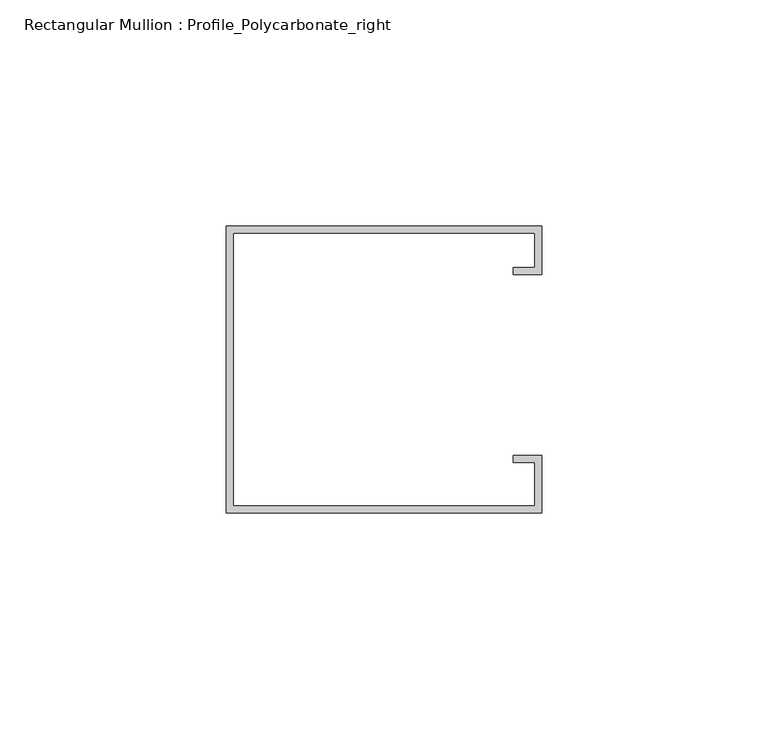
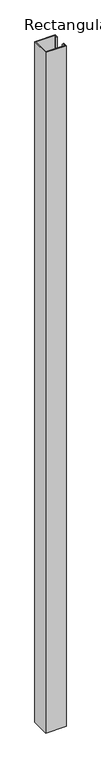
"""IFC4 building model written with IfcOpenShell, lengths in millimetres: member geometry, Rectangular Mullion : Profile_Polycarbonate_right."""

from ifc_helpers import new_model, si_unit, frame, origin, place, context, project, spatial, polyline, outline, extrude, source, transform, mapped, element, save


def rectangular_mullion_profile_polycarbonate_right_a2a6d842(model_context):
    return source(origin(), model_context, "Body", "SweptSolid", [
        extrude(outline(polyline([(0.0, -32.7), (0.0, 30.8), (69.85, 30.8), (69.85, 20.0), (63.5, 20.0), (63.5, 21.5875), (68.2625, 21.5875), (68.2625, 29.2125), (1.5875, 29.2125), (1.5875, -31.1125), (68.2625, -31.1125), (68.2625, -21.5875), (63.5, -21.5875), (63.5, -20.0), (69.85, -20.0), (69.85, -32.7), (0.0, -32.7)])), frame((0.0, 0.0, -2461.6132885), z_axis=(0.0, 0.0, 1.0), x_axis=(1.0, 0.0, 0.0)), (0.0, 0.0, 1.0), 2461.6132885),
    ])


if __name__ == "__main__":
    model = new_model("IFC4")
    model_context = context("Model", 3, world=origin())
    ifc_project = project(units=[si_unit("LENGTHUNIT", "METRE", prefix="MILLI")], contexts=[model_context])
    site = spatial("IfcSite", under=ifc_project)
    building = spatial("IfcBuilding", under=site)
    placement = place(None, origin())
    rectangular_mullion_profile_polycarbonate_right_shape = rectangular_mullion_profile_polycarbonate_right_a2a6d842(model_context)
    element("IfcMember", 1, ObjectType="Rectangular Mullion : Profile_Polycarbonate_right", at=placement, inside=building, context=model_context, shape_type="MappedRepresentation", body=[
        mapped(rectangular_mullion_profile_polycarbonate_right_shape, transform((0.0, 0.0, 0.0), x_axis=(1.0, 0.0, 0.0), y_axis=(0.0, 1.0, 0.0), z_axis=(0.0, 0.0, 1.0))),
    ])
    save(model, "model.ifc")

# Revit data of these elements
# Type "Rectangular Mullion : Profile_Polycarbonate_right"
#   built-in parameter 1007322 = 0.208333 (stored number, unit not read)
#   built-in parameter 1007321 = 0 (stored number, unit not read)
#   built-in parameter 1007320 = 0.00520833 (stored number, unit not read)
# Element 1 (IfcMember, "Rectangular Mullion : Profile_Polycarbonate_right")
#   Materials on its faces: "ALUMINUM PROFILE AT POLYCARBONATE PANEL"
# Materials
#   "ALUMINUM PROFILE AT POLYCARBONATE PANEL": class "Metal", colour RGB 244 244 244, transparency 0, Description = "Aluminum 6061", Cost = 0
